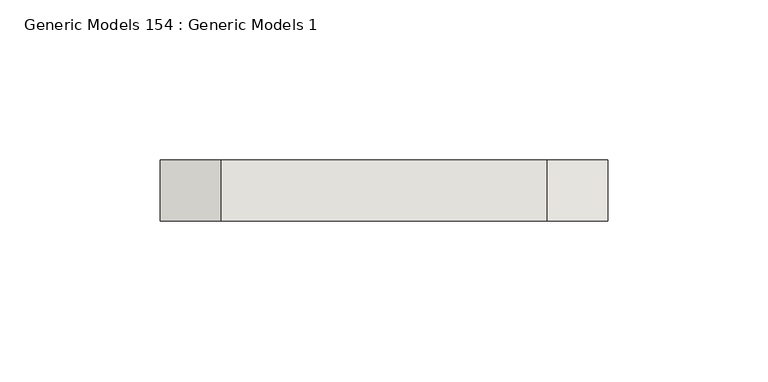
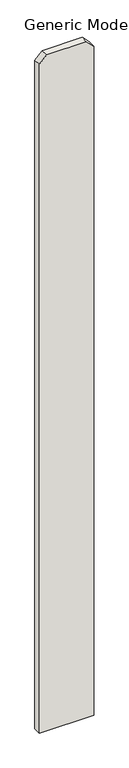
"""IFC4 building model written with IfcOpenShell, lengths in millimetres: wall geometry, Generic Models 154 : Generic Models 1."""

import ifcopenshell
import ifcopenshell.guid

model = None  # the IFC model being written
_history = None  # IfcOwnerHistory: only IFC2X3 demands one
_inside = {}  # id of a spatial element -> (the spatial element, [elements in it])
_under = {}  # id of a project, library or spatial element -> (it, [spatial elements below it])
_declared = {}  # id of a project -> (the project, [libraries it declares])
_typed = {}  # id of a type object -> (the type object, [elements of that type])
_made_of = {}  # id of a material, layer set ... -> (it, [elements and type objects made of it])


def new_model(schema):
    """Start an empty IFC model of exactly this schema.

    Asked for "IFC4X3", IfcOpenShell would pick the latest addendum, in which some entities
    have other attributes; the version numbers below select the first issue.
    IFC2X3 requires an IfcOwnerHistory on every rooted entity: one is made here for all.
    """
    global model, _history
    if schema == "IFC4X3":
        model = ifcopenshell.file(schema_version=(4, 3, 0, 0))
    else:
        model = ifcopenshell.file(schema=schema)
    _inside.clear()
    _under.clear()
    _declared.clear()
    _typed.clear()
    _made_of.clear()
    _history = None
    if model.schema == "IFC2X3":
        org = make("IfcOrganization", Name="unknown")
        user = make(
            "IfcPersonAndOrganization",
            ThePerson=make("IfcPerson", FamilyName="unknown"),
            TheOrganization=org,
        )
        app = make(
            "IfcApplication",
            ApplicationDeveloper=org,
            Version="unknown",
            ApplicationFullName="unknown",
            ApplicationIdentifier="unknown",
        )
        _history = make(
            "IfcOwnerHistory",
            OwningUser=user,
            OwningApplication=app,
            ChangeAction="ADDED",
            CreationDate=0,
        )
    return model


def make(cls, **values):
    """One entity of the class cls with the attributes given. An attribute that is None is left unset."""
    return model.create_entity(
        cls, **{name: value for name, value in values.items() if value is not None}
    )


def rooted(cls, **values):
    """An entity with a GlobalId (a new one), such as an element, a storey or a relation."""
    return make(cls, GlobalId=ifcopenshell.guid.new(), OwnerHistory=_history, **values)


def si_unit(unit_type, name, prefix=None):
    """IfcSIUnit, for example si_unit("LENGTHUNIT", "METRE", prefix="MILLI")."""
    return make("IfcSIUnit", UnitType=unit_type, Prefix=prefix, Name=name)


def assignment(units):
    """IfcUnitAssignment: the units of a project."""
    return None if units is None else make("IfcUnitAssignment", Units=units)


def point(xyz):
    """IfcCartesianPoint."""
    return None if xyz is None else make("IfcCartesianPoint", Coordinates=xyz)


def direction(xyz):
    """IfcDirection."""
    return None if xyz is None else make("IfcDirection", DirectionRatios=xyz)


def frame(location, z_axis=None, x_axis=None):
    """IfcAxis2Placement3D, a coordinate frame: its origin and axes. An axis left out is left unset."""
    return make(
        "IfcAxis2Placement3D",
        Location=point(location),
        Axis=direction(z_axis),
        RefDirection=direction(x_axis),
    )


def origin():
    """The frame at (0, 0, 0) with its axes left unset."""
    return frame((0.0, 0.0, 0.0))


def place(relative_to, where):
    """IfcLocalPlacement: puts the frame where relative to a parent placement (None: the world)."""
    return make(
        "IfcLocalPlacement", PlacementRelTo=relative_to, RelativePlacement=where
    )


def context(
    kind, dimensions, precision=None, world=None, true_north=None, identifier=None
):
    """IfcGeometricRepresentationContext, for example the 3D "Model" context."""
    return make(
        "IfcGeometricRepresentationContext",
        ContextIdentifier=identifier,
        ContextType=kind,
        CoordinateSpaceDimension=dimensions,
        Precision=precision,
        WorldCoordinateSystem=world,
        TrueNorth=true_north,
    )


def project(units=None, contexts=None):
    """IfcProject with its units and contexts."""
    return rooted(
        "IfcProject",
        Name="project",
        RepresentationContexts=contexts,
        UnitsInContext=assignment(units),
    )


def spatial(cls, under=None, at=None, **own):
    """A site, building, storey or space (cls), placed at a placement, below another one or the project."""
    s = rooted(cls, ObjectPlacement=at, **own)
    if under is not None:
        _under.setdefault(under.id(), (under, []))[1].append(s)
    return s


def polyline(points):
    """IfcPolyline through the points."""
    return make("IfcPolyline", Points=[point(p) for p in points])


def outline(outer, holes=None, kind="AREA"):
    """IfcArbitraryClosedProfileDef: a profile drawn as a closed curve; with holes, ...WithVoids."""
    if holes is None:
        return make("IfcArbitraryClosedProfileDef", ProfileType=kind, OuterCurve=outer)
    return make(
        "IfcArbitraryProfileDefWithVoids",
        ProfileType=kind,
        OuterCurve=outer,
        InnerCurves=holes,
    )


def extrude(swept, where, along, depth):
    """IfcExtrudedAreaSolid: the profile swept, set in the frame where, extruded along a direction by depth."""
    return make(
        "IfcExtrudedAreaSolid",
        SweptArea=swept,
        Position=where,
        ExtrudedDirection=direction(along),
        Depth=depth,
    )


def shape(context_of_items, identifier, shape_type, items):
    """IfcShapeRepresentation: the items that make up one representation, for example the "Body"."""
    return make(
        "IfcShapeRepresentation",
        ContextOfItems=context_of_items,
        RepresentationIdentifier=identifier,
        RepresentationType=shape_type,
        Items=items,
    )


def source(mapping_origin, context_of_items, identifier, shape_type, items):
    """IfcRepresentationMap: a shape defined once, which mapped items show again and again."""
    return make(
        "IfcRepresentationMap",
        MappingOrigin=mapping_origin,
        MappedRepresentation=shape(context_of_items, identifier, shape_type, items),
    )


def transform(
    local_origin,
    x_axis=None,
    y_axis=None,
    z_axis=None,
    scale=None,
    scale2=None,
    scale3=None,
    uniform=True,
):
    """IfcCartesianTransformationOperator3D, or its non-uniform kind. x_axis, y_axis, z_axis: its Axis1, 2, 3."""
    if uniform:
        return make(
            "IfcCartesianTransformationOperator3D",
            Axis1=direction(x_axis),
            Axis2=direction(y_axis),
            LocalOrigin=point(local_origin),
            Scale=scale,
            Axis3=direction(z_axis),
        )
    return make(
        "IfcCartesianTransformationOperator3DnonUniform",
        Axis1=direction(x_axis),
        Axis2=direction(y_axis),
        LocalOrigin=point(local_origin),
        Scale=scale,
        Axis3=direction(z_axis),
        Scale2=scale2,
        Scale3=scale3,
    )


def mapped(mapping_source, mapping_target):
    """IfcMappedItem: shows the shape of a source again, moved by a transform."""
    return make(
        "IfcMappedItem", MappingSource=mapping_source, MappingTarget=mapping_target
    )


def made_of(thing, what):
    """Note that an element or type object is made of a material, layer set ...; save() writes the relation."""
    if what is not None:
        _made_of.setdefault(what.id(), (what, []))[1].append(thing)
    return thing


def element(
    cls,
    number,
    at=None,
    inside=None,
    cuts=None,
    type_object=None,
    material=None,
    context=None,
    identifier="Body",
    shape_type=None,
    held_by="IfcProductDefinitionShape",
    body=None,
    shapes=None,
    **own,
):
    """One element of the class cls, such as IfcWall. Its Tag is "e" and its number.

    at: its placement. inside: the storey or other place that contains it. cuts: it is an
    opening in that element (IfcRelVoidsElement). A single representation is given by context,
    identifier, shape_type and body (its items); several are given by shapes. held_by: the class
    of the entity that holds the representations. save() writes the other relations.
    """
    e = rooted(cls, Tag="e%d" % number, ObjectPlacement=at, **own)
    if body is not None:
        shapes = [shape(context, identifier, shape_type, body)]
    if shapes is not None:
        e.Representation = make(held_by, Representations=shapes)
    if inside is not None:
        _inside.setdefault(inside.id(), (inside, []))[1].append(e)
    if cuts is not None:
        rooted(
            "IfcRelVoidsElement", RelatingBuildingElement=cuts, RelatedOpeningElement=e
        )
    if type_object is not None:
        _typed.setdefault(type_object.id(), (type_object, []))[1].append(e)
    return made_of(e, material)


def aggregate(whole, parts):
    """IfcRelAggregates: a whole, such as a stair, and the parts it consists of."""
    return rooted("IfcRelAggregates", RelatingObject=whole, RelatedObjects=parts)


def save(model, path):
    """Write the relations noted so far, then the file.

    IfcRelAggregates (storeys below a building ...), IfcRelContainedInSpatialStructure (elements
    in a storey), IfcRelDefinesByType, IfcRelAssociatesMaterial and IfcRelDeclares: one each for
    every whole, place, type object, material and project.
    """
    for whole, parts in _under.values():
        aggregate(whole, parts)
    for where, things in _inside.values():
        rooted(
            "IfcRelContainedInSpatialStructure",
            RelatedElements=things,
            RelatingStructure=where,
        )
    for kind, things in _typed.values():
        rooted("IfcRelDefinesByType", RelatedObjects=things, RelatingType=kind)
    for what, things in _made_of.values():
        rooted("IfcRelAssociatesMaterial", RelatedObjects=things, RelatingMaterial=what)
    for by, libraries in _declared.values():
        rooted("IfcRelDeclares", RelatingContext=by, RelatedDefinitions=libraries)
    model.write(path)


def generic_models_154_generic_models_1_edaf7e58(model_context):
    return source(origin(), model_context, "Body", "SweptSolid", [
        extrude(outline(polyline([(76.2, 322908.6125), (1885.95, 322908.6125), (1905.0, 322889.5625), (1905.0, 322787.9625), (1885.95, 322768.9125), (76.2, 322768.9125), (76.2, 322908.6125)])), frame((0.0, 547.6875, 0.0), z_axis=(0.0, 1.0, 0.0), x_axis=(0.0, 0.0, 1.0)), (0.0, 0.0, 1.0), 19.05),
    ])


if __name__ == "__main__":
    model = new_model("IFC4")
    model_context = context("Model", 3, world=origin())
    ifc_project = project(units=[si_unit("LENGTHUNIT", "METRE", prefix="MILLI")], contexts=[model_context])
    site = spatial("IfcSite", under=ifc_project)
    building = spatial("IfcBuilding", under=site)
    placement = place(None, origin())
    generic_models_154_generic_models_1_shape = generic_models_154_generic_models_1_edaf7e58(model_context)
    element("IfcWall", 1, ObjectType="Generic Models 154 : Generic Models 1", at=placement, inside=building, context=model_context, shape_type="MappedRepresentation", body=[
        mapped(generic_models_154_generic_models_1_shape, transform((0.0, 0.0, 0.0), x_axis=(1.0, 0.0, 0.0), y_axis=(0.0, 1.0, 0.0), z_axis=(0.0, 0.0, 1.0))),
    ])
    save(model, "model.ifc")

# Revit data of these elements
# Element 1 (IfcWall, "Generic Models 154 : Generic Models 1")
#   Materials on its faces: "VERTICAL 1X6 CEDAR PLANKS W/ CLEAR WOOD SEALER"
# Materials
#   "VERTICAL 1X6 CEDAR PLANKS W/ CLEAR WOOD SEALER": class "Wood", colour RGB 234 198 147, transparency 0, Description = "Pinus Echinata", Cost = 0
